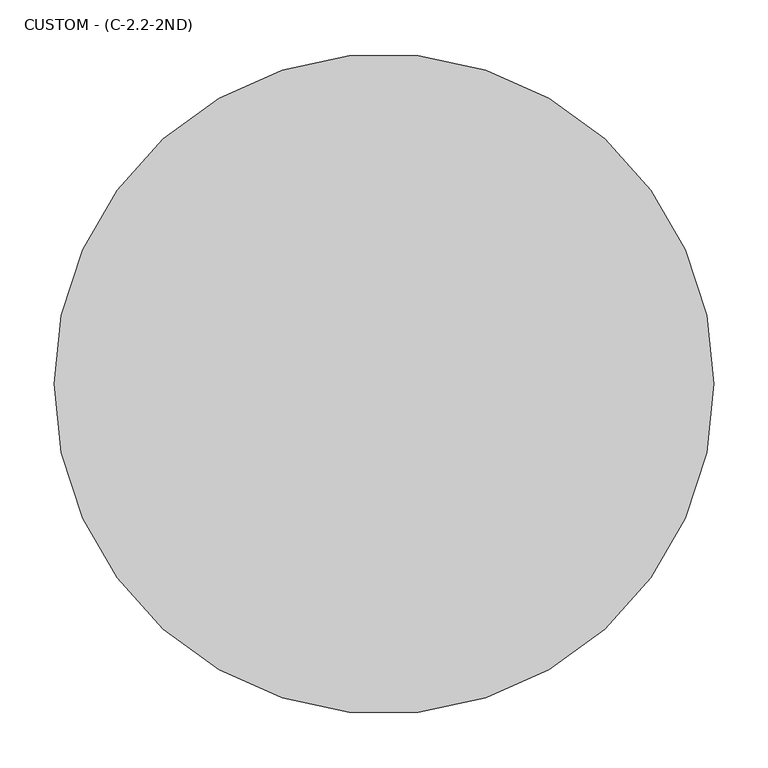
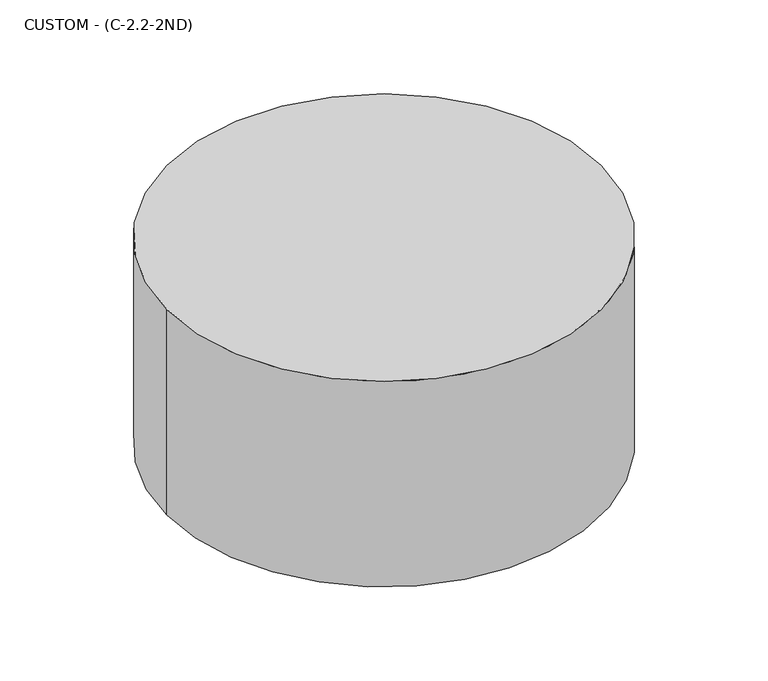
"""IFC4 building model written with IfcOpenShell, lengths in millimetres: fastener geometry, Sturctural Connector - Placeholder : CUSTOM - (C-2.2-2ND)."""

from ifc_helpers import new_model, si_unit, point, origin, origin_with_axes, origin_2d, place, context, project, spatial, circle_curve, trimmed, segment, composite_curve, outline, extrude, source, transform, mapped, element, save


def custom_c_2_2_2nd_84da08ab(model_context):
    return source(origin(), model_context, "Body", "SweptSolid", [
        extrude(outline(composite_curve([segment(trimmed(circle_curve(origin_2d(), 304.8), [point((-304.8, 0.0))], [point((304.8, 0.0))], False, "CARTESIAN"), True, "CONTINUOUS"), segment(trimmed(circle_curve(origin_2d(), 304.8), [point((304.8, 0.0))], [point((-304.8, 0.0))], False, "CARTESIAN"), True, "CONTINUOUS")], self_intersect=False)), origin_with_axes(), (0.0, 0.0, 1.0), 304.8),
    ])


if __name__ == "__main__":
    model = new_model("IFC4")
    model_context = context("Model", 3, world=origin())
    ifc_project = project(units=[si_unit("LENGTHUNIT", "METRE", prefix="MILLI")], contexts=[model_context])
    site = spatial("IfcSite", under=ifc_project)
    building = spatial("IfcBuilding", under=site)
    placement = place(None, origin())
    custom_c_2_2_2nd_shape = custom_c_2_2_2nd_84da08ab(model_context)
    element("IfcFastener", 1, ObjectType="Sturctural Connector - Placeholder : CUSTOM - (C-2.2-2ND)", at=placement, inside=building, context=model_context, shape_type="MappedRepresentation", body=[
        mapped(custom_c_2_2_2nd_shape, transform((0.0, 0.0, 0.0), x_axis=(1.0, 0.0, 0.0), y_axis=(0.0, 1.0, 0.0), z_axis=(0.0, 0.0, 1.0))),
    ])
    save(model, "model.ifc")
